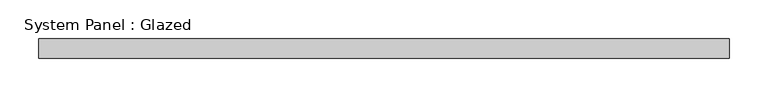
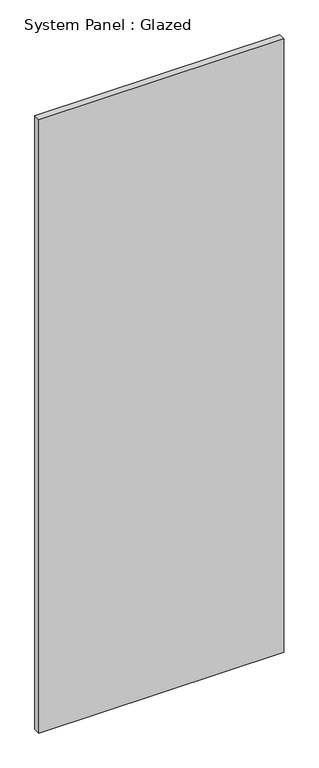
"""IFC4 building model written with IfcOpenShell, lengths in millimetres: plate geometry, System Panel : Glazed."""

from ifc_helpers import new_model, si_unit, origin, origin_with_axes, place, context, project, spatial, polyline, outline, extrude, source, transform, mapped, element, save


def system_panel_glazed_137828db(model_context):
    return source(origin(), model_context, "Body", "SweptSolid", [
        extrude(outline(polyline([(443.75, 24.5), (-443.75, 24.5), (-443.75, 49.5), (443.75, 49.5), (443.75, 24.5)])), origin_with_axes(), (0.0, 0.0, 1.0), 2350.0),
    ])


if __name__ == "__main__":
    model = new_model("IFC4")
    model_context = context("Model", 3, world=origin())
    ifc_project = project(units=[si_unit("LENGTHUNIT", "METRE", prefix="MILLI")], contexts=[model_context])
    site = spatial("IfcSite", under=ifc_project)
    building = spatial("IfcBuilding", under=site)
    placement = place(None, origin())
    system_panel_glazed_shape = system_panel_glazed_137828db(model_context)
    element("IfcPlate", 1, ObjectType="System Panel : Glazed", at=placement, inside=building, context=model_context, shape_type="MappedRepresentation", body=[
        mapped(system_panel_glazed_shape, transform((0.0, 0.0, 0.0), x_axis=(1.0, 0.0, 0.0), y_axis=(0.0, 1.0, 0.0), z_axis=(0.0, 0.0, 1.0))),
    ])
    save(model, "model.ifc")

# Revit data of these elements
# Type "System Panel : Glazed"
#   Construction Type Id = "GSP4R"
#   Analytic Construction = "1/8 in Pilkington single glazing"
#   Visual Light Transmittance = 0.9
#   Solar Heat Gain Coefficient = 0.86
#   Heat Transfer Coefficient (U) = 6.7069 W/(m²·K)
#   Define Thermal Properties by = 1
# Element 1 (IfcPlate, "System Panel : Glazed")
#   Materials on its faces: "Glass"
# Materials
#   "Glass": class "Glass", colour RGB 0 128 192, transparency 0.9, Description = "Soda Lime Glass", Cost = 0
